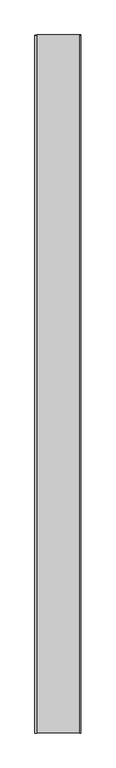
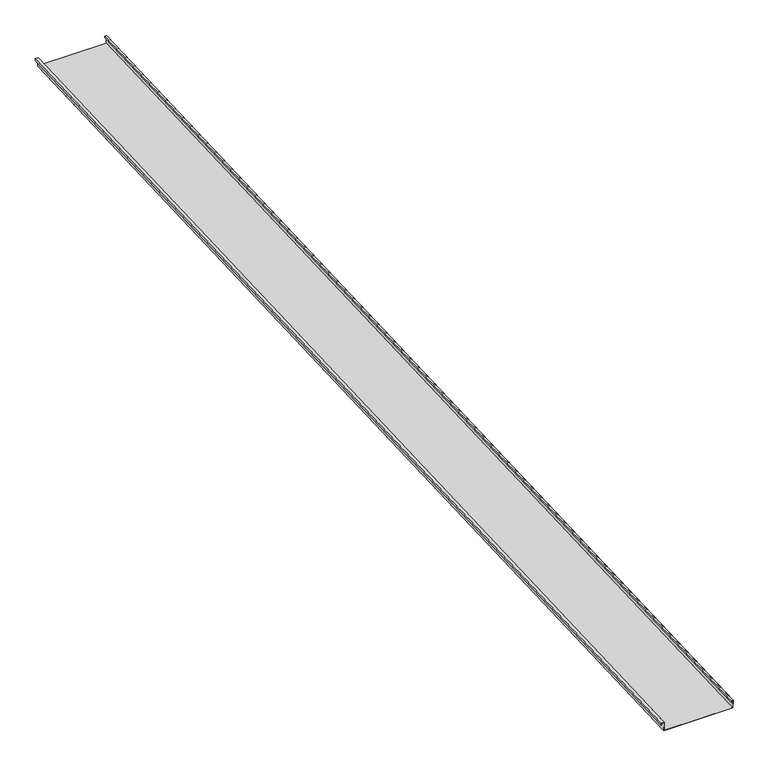
"""IFC4 building model written with IfcOpenShell, lengths in millimetres: proxy geometry, Generic Models 2:Generic Models 2:310765:Generic Models 2:310765 : Generic Models 2:Generic Models 2:310765:94 : Generic Models 2:Generic Models 2:310765:Generic Models 2:310765 : Generic Models 2:Generic Models 2:310765:300385."""

import ifcopenshell
import ifcopenshell.guid

model = None  # the IFC model being written
_history = None  # IfcOwnerHistory: only IFC2X3 demands one
_inside = {}  # id of a spatial element -> (the spatial element, [elements in it])
_under = {}  # id of a project, library or spatial element -> (it, [spatial elements below it])
_declared = {}  # id of a project -> (the project, [libraries it declares])
_typed = {}  # id of a type object -> (the type object, [elements of that type])
_made_of = {}  # id of a material, layer set ... -> (it, [elements and type objects made of it])


def new_model(schema):
    """Start an empty IFC model of exactly this schema.

    Asked for "IFC4X3", IfcOpenShell would pick the latest addendum, in which some entities
    have other attributes; the version numbers below select the first issue.
    IFC2X3 requires an IfcOwnerHistory on every rooted entity: one is made here for all.
    """
    global model, _history
    if schema == "IFC4X3":
        model = ifcopenshell.file(schema_version=(4, 3, 0, 0))
    else:
        model = ifcopenshell.file(schema=schema)
    _inside.clear()
    _under.clear()
    _declared.clear()
    _typed.clear()
    _made_of.clear()
    _history = None
    if model.schema == "IFC2X3":
        org = make("IfcOrganization", Name="unknown")
        user = make(
            "IfcPersonAndOrganization",
            ThePerson=make("IfcPerson", FamilyName="unknown"),
            TheOrganization=org,
        )
        app = make(
            "IfcApplication",
            ApplicationDeveloper=org,
            Version="unknown",
            ApplicationFullName="unknown",
            ApplicationIdentifier="unknown",
        )
        _history = make(
            "IfcOwnerHistory",
            OwningUser=user,
            OwningApplication=app,
            ChangeAction="ADDED",
            CreationDate=0,
        )
    return model


def make(cls, **values):
    """One entity of the class cls with the attributes given. An attribute that is None is left unset."""
    return model.create_entity(
        cls, **{name: value for name, value in values.items() if value is not None}
    )


def rooted(cls, **values):
    """An entity with a GlobalId (a new one), such as an element, a storey or a relation."""
    return make(cls, GlobalId=ifcopenshell.guid.new(), OwnerHistory=_history, **values)


def si_unit(unit_type, name, prefix=None):
    """IfcSIUnit, for example si_unit("LENGTHUNIT", "METRE", prefix="MILLI")."""
    return make("IfcSIUnit", UnitType=unit_type, Prefix=prefix, Name=name)


def assignment(units):
    """IfcUnitAssignment: the units of a project."""
    return None if units is None else make("IfcUnitAssignment", Units=units)


def point(xyz):
    """IfcCartesianPoint."""
    return None if xyz is None else make("IfcCartesianPoint", Coordinates=xyz)


def direction(xyz):
    """IfcDirection."""
    return None if xyz is None else make("IfcDirection", DirectionRatios=xyz)


def frame(location, z_axis=None, x_axis=None):
    """IfcAxis2Placement3D, a coordinate frame: its origin and axes. An axis left out is left unset."""
    return make(
        "IfcAxis2Placement3D",
        Location=point(location),
        Axis=direction(z_axis),
        RefDirection=direction(x_axis),
    )


def origin():
    """The frame at (0, 0, 0) with its axes left unset."""
    return frame((0.0, 0.0, 0.0))


def place(relative_to, where):
    """IfcLocalPlacement: puts the frame where relative to a parent placement (None: the world)."""
    return make(
        "IfcLocalPlacement", PlacementRelTo=relative_to, RelativePlacement=where
    )


def context(
    kind, dimensions, precision=None, world=None, true_north=None, identifier=None
):
    """IfcGeometricRepresentationContext, for example the 3D "Model" context."""
    return make(
        "IfcGeometricRepresentationContext",
        ContextIdentifier=identifier,
        ContextType=kind,
        CoordinateSpaceDimension=dimensions,
        Precision=precision,
        WorldCoordinateSystem=world,
        TrueNorth=true_north,
    )


def project(units=None, contexts=None):
    """IfcProject with its units and contexts."""
    return rooted(
        "IfcProject",
        Name="project",
        RepresentationContexts=contexts,
        UnitsInContext=assignment(units),
    )


def spatial(cls, under=None, at=None, **own):
    """A site, building, storey or space (cls), placed at a placement, below another one or the project."""
    s = rooted(cls, ObjectPlacement=at, **own)
    if under is not None:
        _under.setdefault(under.id(), (under, []))[1].append(s)
    return s


def polyline(points):
    """IfcPolyline through the points."""
    return make("IfcPolyline", Points=[point(p) for p in points])


def outline(outer, holes=None, kind="AREA"):
    """IfcArbitraryClosedProfileDef: a profile drawn as a closed curve; with holes, ...WithVoids."""
    if holes is None:
        return make("IfcArbitraryClosedProfileDef", ProfileType=kind, OuterCurve=outer)
    return make(
        "IfcArbitraryProfileDefWithVoids",
        ProfileType=kind,
        OuterCurve=outer,
        InnerCurves=holes,
    )


def extrude(swept, where, along, depth):
    """IfcExtrudedAreaSolid: the profile swept, set in the frame where, extruded along a direction by depth."""
    return make(
        "IfcExtrudedAreaSolid",
        SweptArea=swept,
        Position=where,
        ExtrudedDirection=direction(along),
        Depth=depth,
    )


def shape(context_of_items, identifier, shape_type, items):
    """IfcShapeRepresentation: the items that make up one representation, for example the "Body"."""
    return make(
        "IfcShapeRepresentation",
        ContextOfItems=context_of_items,
        RepresentationIdentifier=identifier,
        RepresentationType=shape_type,
        Items=items,
    )


def source(mapping_origin, context_of_items, identifier, shape_type, items):
    """IfcRepresentationMap: a shape defined once, which mapped items show again and again."""
    return make(
        "IfcRepresentationMap",
        MappingOrigin=mapping_origin,
        MappedRepresentation=shape(context_of_items, identifier, shape_type, items),
    )


def transform(
    local_origin,
    x_axis=None,
    y_axis=None,
    z_axis=None,
    scale=None,
    scale2=None,
    scale3=None,
    uniform=True,
):
    """IfcCartesianTransformationOperator3D, or its non-uniform kind. x_axis, y_axis, z_axis: its Axis1, 2, 3."""
    if uniform:
        return make(
            "IfcCartesianTransformationOperator3D",
            Axis1=direction(x_axis),
            Axis2=direction(y_axis),
            LocalOrigin=point(local_origin),
            Scale=scale,
            Axis3=direction(z_axis),
        )
    return make(
        "IfcCartesianTransformationOperator3DnonUniform",
        Axis1=direction(x_axis),
        Axis2=direction(y_axis),
        LocalOrigin=point(local_origin),
        Scale=scale,
        Axis3=direction(z_axis),
        Scale2=scale2,
        Scale3=scale3,
    )


def mapped(mapping_source, mapping_target):
    """IfcMappedItem: shows the shape of a source again, moved by a transform."""
    return make(
        "IfcMappedItem", MappingSource=mapping_source, MappingTarget=mapping_target
    )


def made_of(thing, what):
    """Note that an element or type object is made of a material, layer set ...; save() writes the relation."""
    if what is not None:
        _made_of.setdefault(what.id(), (what, []))[1].append(thing)
    return thing


def element(
    cls,
    number,
    at=None,
    inside=None,
    cuts=None,
    type_object=None,
    material=None,
    context=None,
    identifier="Body",
    shape_type=None,
    held_by="IfcProductDefinitionShape",
    body=None,
    shapes=None,
    **own,
):
    """One element of the class cls, such as IfcWall. Its Tag is "e" and its number.

    at: its placement. inside: the storey or other place that contains it. cuts: it is an
    opening in that element (IfcRelVoidsElement). A single representation is given by context,
    identifier, shape_type and body (its items); several are given by shapes. held_by: the class
    of the entity that holds the representations. save() writes the other relations.
    """
    e = rooted(cls, Tag="e%d" % number, ObjectPlacement=at, **own)
    if body is not None:
        shapes = [shape(context, identifier, shape_type, body)]
    if shapes is not None:
        e.Representation = make(held_by, Representations=shapes)
    if inside is not None:
        _inside.setdefault(inside.id(), (inside, []))[1].append(e)
    if cuts is not None:
        rooted(
            "IfcRelVoidsElement", RelatingBuildingElement=cuts, RelatedOpeningElement=e
        )
    if type_object is not None:
        _typed.setdefault(type_object.id(), (type_object, []))[1].append(e)
    return made_of(e, material)


def aggregate(whole, parts):
    """IfcRelAggregates: a whole, such as a stair, and the parts it consists of."""
    return rooted("IfcRelAggregates", RelatingObject=whole, RelatedObjects=parts)


def save(model, path):
    """Write the relations noted so far, then the file.

    IfcRelAggregates (storeys below a building ...), IfcRelContainedInSpatialStructure (elements
    in a storey), IfcRelDefinesByType, IfcRelAssociatesMaterial and IfcRelDeclares: one each for
    every whole, place, type object, material and project.
    """
    for whole, parts in _under.values():
        aggregate(whole, parts)
    for where, things in _inside.values():
        rooted(
            "IfcRelContainedInSpatialStructure",
            RelatedElements=things,
            RelatingStructure=where,
        )
    for kind, things in _typed.values():
        rooted("IfcRelDefinesByType", RelatedObjects=things, RelatingType=kind)
    for what, things in _made_of.values():
        rooted("IfcRelAssociatesMaterial", RelatedObjects=things, RelatingMaterial=what)
    for by, libraries in _declared.values():
        rooted("IfcRelDeclares", RelatingContext=by, RelatedDefinitions=libraries)
    model.write(path)


def generic_models_0283b779(model_context):
    return source(origin(), model_context, "Body", "SweptSolid", [
        extrude(outline(polyline([(1.5875, 0.0), (1.5875, 50.8), (407.9875, 50.8), (407.9875, 1.5875), (396.875, 1.5875), (396.875, 11.1125), (398.4625, 11.1125), (398.4625, 3.175), (406.4, 3.175), (406.4, 49.2125), (3.175, 49.2125), (3.175, -1.5874999), (-14.2875, -1.5874999), (-14.2875, 9.525), (-12.7, 9.525), (-12.7, 0.0), (1.5875, 0.0)])), frame((614779.0763073, -581354.4345603, 3902.6697972), z_axis=(0.0, 0.9991330730923568, 0.041630544712067834), x_axis=(1.0, 0.0, 0.0)), (0.0, 0.0, 1.0), 6400.8),
    ])


if __name__ == "__main__":
    model = new_model("IFC4")
    model_context = context("Model", 3, world=origin())
    ifc_project = project(units=[si_unit("LENGTHUNIT", "METRE", prefix="MILLI")], contexts=[model_context])
    site = spatial("IfcSite", under=ifc_project)
    building = spatial("IfcBuilding", under=site)
    placement = place(None, origin())
    generic_models_shape = generic_models_0283b779(model_context)
    element("IfcBuildingElementProxy", 1, Name="Generic Models 2:Generic Models 2:310765:Generic Models 2:310765 : Generic Models 2:Generic Models 2:310765:94 : Generic Models 2:Generic Models 2:310765:Generic Models 2:310765 : Generic Models 2:Generic Models 2:310765:300385", ObjectType="Generic Models 2:Generic Models 2:310765:Generic Models 2:310765 : Generic Models 2:Generic Models 2:310765:94 : Generic Models 2:Generic Models 2:310765:Generic Models 2:310765 : Generic Models 2:Generic Models 2:310765:300385", at=placement, inside=building, context=model_context, shape_type="MappedRepresentation", body=[
        mapped(generic_models_shape, transform((0.0, 0.0, 0.0), x_axis=(1.0, 0.0, 0.0), y_axis=(0.0, 1.0, 0.0), z_axis=(0.0, 0.0, 1.0))),
    ])
    save(model, "model.ifc")

# Revit data of these elements
# Project information
#   IfcSite GUID = "2naYFwtnGHv906093rt3ko"
#   IfcBuilding GUID = "2naZIetnGHv906093rt3ko"
#   IfcProject GUID = "5efaeb93_8b82_4a45_8c7"
#   NumberOfStoreys = "1"
#   NameOverride = "Default"
#   Project Issue Date = "Issue Date"
#   Project Status = "Project Status"
#   Client Name = "Owner"
#   Project Address = "Enter address here"
#   Project Name = "Project Name"
#   Project Number = "Project Number"
# Type "Generic Models 2:Generic Models 2:310765:Generic Models 2:310765 : Generic Models 2:Generic Models 2:310765:94 : Generic Models 2:Generic Models 2:310765:Generic Models 2:310765 : Generic Models 2:Generic Models 2:310765:300385"
#   NameOverride = "Generic Models 2:Generic Models 2:310765:Generic Models 2:310765 : Generic Models 2:Generic Models 2:310765:300385"
#   ObjectTypeOverride = "Generic Models 2:310765 : Generic Models 2:Generic Models 2:310765"
#   Reference = "Generic Models 2"
#   Tag = "300385"
# Element 1 (IfcBuildingElementProxy, "Generic Models 2:Generic Models 2:310765:Generic Models 2:310765 : Generic Models 2:Generic Models 2:310765:94 : Generic Models 2:Generic Models 2:310765:Generic Models 2:310765 : Generic Models 2:Generic Models 2:310765:300385")
#   Materials on its faces: "THERMAL BROKEN ALUMINUM STOREFRONT FOR POLYCARBONATE"
# Materials
#   "THERMAL BROKEN ALUMINUM STOREFRONT FOR POLYCARBONATE": class "Unassigned", colour RGB 244 244 244, transparency 0, Keynote = "M07611300.01", Cost = 0
